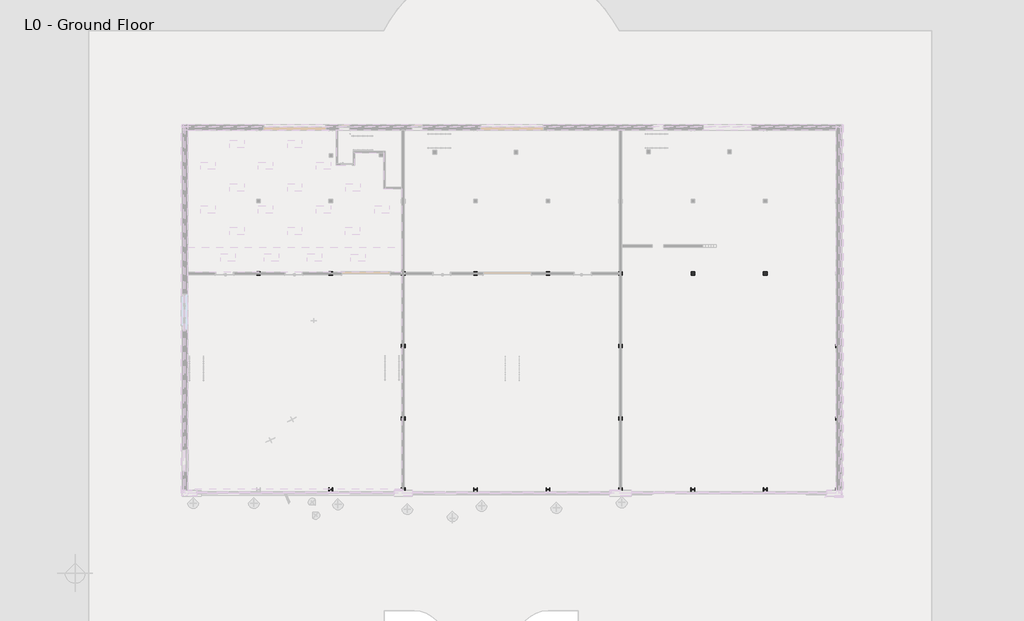
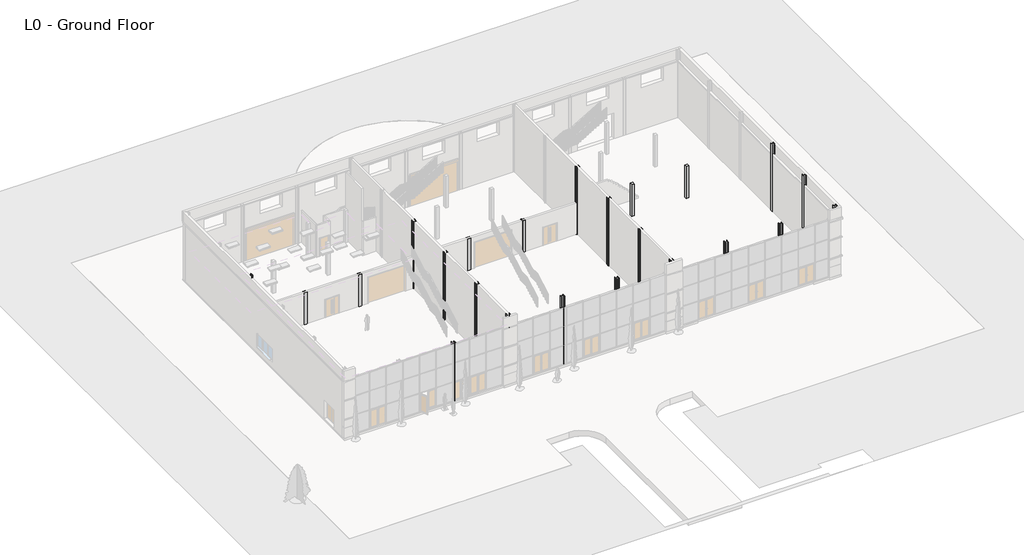
# One storey, part 6 of 14: 23 columns, 22 slabs, 8 footings.
"""IFC4 building model written with IfcOpenShell, lengths in millimetres."""

import ifcopenshell
import ifcopenshell.guid

model = None  # the IFC model being written
_history = None  # IfcOwnerHistory: only IFC2X3 demands one
_inside = {}  # id of a spatial element -> (the spatial element, [elements in it])
_under = {}  # id of a project, library or spatial element -> (it, [spatial elements below it])
_declared = {}  # id of a project -> (the project, [libraries it declares])
_typed = {}  # id of a type object -> (the type object, [elements of that type])
_made_of = {}  # id of a material, layer set ... -> (it, [elements and type objects made of it])


def new_model(schema):
    """Start an empty IFC model of exactly this schema.

    Asked for "IFC4X3", IfcOpenShell would pick the latest addendum, in which some entities
    have other attributes; the version numbers below select the first issue.
    IFC2X3 requires an IfcOwnerHistory on every rooted entity: one is made here for all.
    """
    global model, _history
    if schema == "IFC4X3":
        model = ifcopenshell.file(schema_version=(4, 3, 0, 0))
    else:
        model = ifcopenshell.file(schema=schema)
    _inside.clear()
    _under.clear()
    _declared.clear()
    _typed.clear()
    _made_of.clear()
    _history = None
    if model.schema == "IFC2X3":
        org = make("IfcOrganization", Name="unknown")
        user = make(
            "IfcPersonAndOrganization",
            ThePerson=make("IfcPerson", FamilyName="unknown"),
            TheOrganization=org,
        )
        app = make(
            "IfcApplication",
            ApplicationDeveloper=org,
            Version="unknown",
            ApplicationFullName="unknown",
            ApplicationIdentifier="unknown",
        )
        _history = make(
            "IfcOwnerHistory",
            OwningUser=user,
            OwningApplication=app,
            ChangeAction="ADDED",
            CreationDate=0,
        )
    return model


def make(cls, **values):
    """One entity of the class cls with the attributes given. An attribute that is None is left unset."""
    return model.create_entity(
        cls, **{name: value for name, value in values.items() if value is not None}
    )


def rooted(cls, **values):
    """An entity with a GlobalId (a new one), such as an element, a storey or a relation."""
    return make(cls, GlobalId=ifcopenshell.guid.new(), OwnerHistory=_history, **values)


def si_unit(unit_type, name, prefix=None):
    """IfcSIUnit, for example si_unit("LENGTHUNIT", "METRE", prefix="MILLI")."""
    return make("IfcSIUnit", UnitType=unit_type, Prefix=prefix, Name=name)


def assignment(units):
    """IfcUnitAssignment: the units of a project."""
    return None if units is None else make("IfcUnitAssignment", Units=units)


def point(xyz):
    """IfcCartesianPoint."""
    return None if xyz is None else make("IfcCartesianPoint", Coordinates=xyz)


def direction(xyz):
    """IfcDirection."""
    return None if xyz is None else make("IfcDirection", DirectionRatios=xyz)


def frame(location, z_axis=None, x_axis=None):
    """IfcAxis2Placement3D, a coordinate frame: its origin and axes. An axis left out is left unset."""
    return make(
        "IfcAxis2Placement3D",
        Location=point(location),
        Axis=direction(z_axis),
        RefDirection=direction(x_axis),
    )


def frame_2d(location, x_axis=None):
    """IfcAxis2Placement2D, a coordinate frame in the plane: its origin and x axis."""
    return make(
        "IfcAxis2Placement2D", Location=point(location), RefDirection=direction(x_axis)
    )


def origin():
    """The frame at (0, 0, 0) with its axes left unset."""
    return frame((0.0, 0.0, 0.0))


def place(relative_to, where):
    """IfcLocalPlacement: puts the frame where relative to a parent placement (None: the world)."""
    return make(
        "IfcLocalPlacement", PlacementRelTo=relative_to, RelativePlacement=where
    )


def context(
    kind, dimensions, precision=None, world=None, true_north=None, identifier=None
):
    """IfcGeometricRepresentationContext, for example the 3D "Model" context."""
    return make(
        "IfcGeometricRepresentationContext",
        ContextIdentifier=identifier,
        ContextType=kind,
        CoordinateSpaceDimension=dimensions,
        Precision=precision,
        WorldCoordinateSystem=world,
        TrueNorth=true_north,
    )


def project(units=None, contexts=None):
    """IfcProject with its units and contexts."""
    return rooted(
        "IfcProject",
        Name="project",
        RepresentationContexts=contexts,
        UnitsInContext=assignment(units),
    )


def spatial(cls, under=None, at=None, **own):
    """A site, building, storey or space (cls), placed at a placement, below another one or the project."""
    s = rooted(cls, ObjectPlacement=at, **own)
    if under is not None:
        _under.setdefault(under.id(), (under, []))[1].append(s)
    return s


def polyline(points):
    """IfcPolyline through the points."""
    return make("IfcPolyline", Points=[point(p) for p in points])


def circle_curve(where, radius):
    """IfcCircle in the frame where."""
    return make("IfcCircle", Position=where, Radius=radius)


def trimmed(basis, trim1, trim2, sense, master):
    """IfcTrimmedCurve: the piece of a basis curve between two trims."""
    return make(
        "IfcTrimmedCurve",
        BasisCurve=basis,
        Trim1=trim1,
        Trim2=trim2,
        SenseAgreement=sense,
        MasterRepresentation=master,
    )


def segment(curve, same_sense, transition):
    """IfcCompositeCurveSegment."""
    return make(
        "IfcCompositeCurveSegment",
        Transition=transition,
        SameSense=same_sense,
        ParentCurve=curve,
    )


def composite_curve(segments, self_intersect=None):
    """IfcCompositeCurve: segments joined end to end."""
    return make("IfcCompositeCurve", Segments=segments, SelfIntersect=self_intersect)


def outline(outer, holes=None, kind="AREA"):
    """IfcArbitraryClosedProfileDef: a profile drawn as a closed curve; with holes, ...WithVoids."""
    if holes is None:
        return make("IfcArbitraryClosedProfileDef", ProfileType=kind, OuterCurve=outer)
    return make(
        "IfcArbitraryProfileDefWithVoids",
        ProfileType=kind,
        OuterCurve=outer,
        InnerCurves=holes,
    )


def extrude(swept, where, along, depth):
    """IfcExtrudedAreaSolid: the profile swept, set in the frame where, extruded along a direction by depth."""
    return make(
        "IfcExtrudedAreaSolid",
        SweptArea=swept,
        Position=where,
        ExtrudedDirection=direction(along),
        Depth=depth,
    )


def faces_of(points, faces, orient=None, outer=None):
    """IfcFace entities. A face is a list of loops; a loop is a list of indices into points, from 0.

    orient and outer hold one flag for each loop. By default every Orientation is true, the
    first loop of a face is its IfcFaceOuterBound and the others are IfcFaceBound.
    """
    made = []
    for i, loops in enumerate(faces):
        bounds = []
        for j, loop in enumerate(loops):
            is_outer = j == 0 if outer is None else outer[i][j]
            bounds.append(
                make(
                    "IfcFaceOuterBound" if is_outer else "IfcFaceBound",
                    Bound=make("IfcPolyLoop", Polygon=[points[k] for k in loop]),
                    Orientation=True if orient is None else orient[i][j],
                )
            )
        made.append(make("IfcFace", Bounds=bounds))
    return made


def faceted_brep(points, faces, orient=None, outer=None, voids=None):
    """IfcFacetedBrep: a solid bounded by flat faces; with voids (closed shells), ...WithVoids."""
    shared = [point(p) for p in points]
    hull = make("IfcClosedShell", CfsFaces=faces_of(shared, faces, orient, outer))
    if voids is None:
        return make("IfcFacetedBrep", Outer=hull)
    return make(
        "IfcFacetedBrepWithVoids",
        Outer=hull,
        Voids=[
            make(cls, CfsFaces=faces_of(shared, fs, o, b)) for cls, fs, o, b in voids
        ],
    )


def shape(context_of_items, identifier, shape_type, items):
    """IfcShapeRepresentation: the items that make up one representation, for example the "Body"."""
    return make(
        "IfcShapeRepresentation",
        ContextOfItems=context_of_items,
        RepresentationIdentifier=identifier,
        RepresentationType=shape_type,
        Items=items,
    )


def source(mapping_origin, context_of_items, identifier, shape_type, items):
    """IfcRepresentationMap: a shape defined once, which mapped items show again and again."""
    return make(
        "IfcRepresentationMap",
        MappingOrigin=mapping_origin,
        MappedRepresentation=shape(context_of_items, identifier, shape_type, items),
    )


def transform(
    local_origin,
    x_axis=None,
    y_axis=None,
    z_axis=None,
    scale=None,
    scale2=None,
    scale3=None,
    uniform=True,
):
    """IfcCartesianTransformationOperator3D, or its non-uniform kind. x_axis, y_axis, z_axis: its Axis1, 2, 3."""
    if uniform:
        return make(
            "IfcCartesianTransformationOperator3D",
            Axis1=direction(x_axis),
            Axis2=direction(y_axis),
            LocalOrigin=point(local_origin),
            Scale=scale,
            Axis3=direction(z_axis),
        )
    return make(
        "IfcCartesianTransformationOperator3DnonUniform",
        Axis1=direction(x_axis),
        Axis2=direction(y_axis),
        LocalOrigin=point(local_origin),
        Scale=scale,
        Axis3=direction(z_axis),
        Scale2=scale2,
        Scale3=scale3,
    )


def mapped(mapping_source, mapping_target):
    """IfcMappedItem: shows the shape of a source again, moved by a transform."""
    return make(
        "IfcMappedItem", MappingSource=mapping_source, MappingTarget=mapping_target
    )


def made_of(thing, what):
    """Note that an element or type object is made of a material, layer set ...; save() writes the relation."""
    if what is not None:
        _made_of.setdefault(what.id(), (what, []))[1].append(thing)
    return thing


def element(
    cls,
    number,
    at=None,
    inside=None,
    cuts=None,
    type_object=None,
    material=None,
    context=None,
    identifier="Body",
    shape_type=None,
    held_by="IfcProductDefinitionShape",
    body=None,
    shapes=None,
    **own,
):
    """One element of the class cls, such as IfcWall. Its Tag is "e" and its number.

    at: its placement. inside: the storey or other place that contains it. cuts: it is an
    opening in that element (IfcRelVoidsElement). A single representation is given by context,
    identifier, shape_type and body (its items); several are given by shapes. held_by: the class
    of the entity that holds the representations. save() writes the other relations.
    """
    e = rooted(cls, Tag="e%d" % number, ObjectPlacement=at, **own)
    if body is not None:
        shapes = [shape(context, identifier, shape_type, body)]
    if shapes is not None:
        e.Representation = make(held_by, Representations=shapes)
    if inside is not None:
        _inside.setdefault(inside.id(), (inside, []))[1].append(e)
    if cuts is not None:
        rooted(
            "IfcRelVoidsElement", RelatingBuildingElement=cuts, RelatedOpeningElement=e
        )
    if type_object is not None:
        _typed.setdefault(type_object.id(), (type_object, []))[1].append(e)
    return made_of(e, material)


def aggregate(whole, parts):
    """IfcRelAggregates: a whole, such as a stair, and the parts it consists of."""
    return rooted("IfcRelAggregates", RelatingObject=whole, RelatedObjects=parts)


def save(model, path):
    """Write the relations noted so far, then the file.

    IfcRelAggregates (storeys below a building ...), IfcRelContainedInSpatialStructure (elements
    in a storey), IfcRelDefinesByType, IfcRelAssociatesMaterial and IfcRelDeclares: one each for
    every whole, place, type object, material and project.
    """
    for whole, parts in _under.values():
        aggregate(whole, parts)
    for where, things in _inside.values():
        rooted(
            "IfcRelContainedInSpatialStructure",
            RelatedElements=things,
            RelatingStructure=where,
        )
    for kind, things in _typed.values():
        rooted("IfcRelDefinesByType", RelatedObjects=things, RelatingType=kind)
    for what, things in _made_of.values():
        rooted("IfcRelAssociatesMaterial", RelatedObjects=things, RelatingMaterial=what)
    for by, libraries in _declared.values():
        rooted("IfcRelDeclares", RelatingContext=by, RelatedDefinitions=libraries)
    model.write(path)


def uc_universal_column_column_305x305x97uc_f4bfb62a(model_context):
    return source(origin(), model_context, "Body", "SweptSolid", [
        extrude(outline(composite_curve([segment(polyline([(152.65, 153.95), (152.65, 138.55), (20.15, 138.55)]), True, "CONTINUOUS"), segment(trimmed(circle_curve(frame_2d((20.15, 123.35)), 15.2), [point((20.15, 138.55))], [point((4.95, 123.35))], True, "CARTESIAN"), True, "CONTINUOUS"), segment(polyline([(4.95, 123.35), (4.95, -123.35)]), True, "CONTINUOUS"), segment(trimmed(circle_curve(frame_2d((20.15, -123.35)), 15.2), [point((4.95, -123.35))], [point((20.15, -138.55))], True, "CARTESIAN"), True, "CONTINUOUS"), segment(polyline([(20.15, -138.55), (152.65, -138.55), (152.65, -153.95), (-152.65, -153.95), (-152.65, -138.55), (-20.15, -138.55)]), True, "CONTINUOUS"), segment(trimmed(circle_curve(frame_2d((-20.15, -123.35)), 15.2), [point((-20.15, -138.55))], [point((-4.95, -123.35))], True, "CARTESIAN"), True, "CONTINUOUS"), segment(polyline([(-4.95, -123.35), (-4.95, 123.35)]), True, "CONTINUOUS"), segment(trimmed(circle_curve(frame_2d((-20.15, 123.35)), 15.2), [point((-4.95, 123.35))], [point((-20.15, 138.55))], True, "CARTESIAN"), True, "CONTINUOUS"), segment(polyline([(-20.15, 138.55), (-152.65, 138.55), (-152.65, 153.95), (152.65, 153.95)]), True, "CONTINUOUS")], self_intersect=False)), frame((0.0, 0.0, -1500.0), z_axis=(0.0, 0.0, 1.0), x_axis=(1.0, 0.0, 0.0)), (0.0, 0.0, 1.0), 9300.0),
    ])


def uc_universal_column_column_305x305x97uc_8da79b43(model_context):
    return source(origin(), model_context, "Body", "SweptSolid", [
        extrude(outline(composite_curve([segment(polyline([(152.65, -153.95), (-152.65, -153.95), (-152.65, -138.55), (-20.15, -138.55)]), True, "CONTINUOUS"), segment(trimmed(circle_curve(frame_2d((-20.15, -123.35)), 15.2), [point((-20.15, -138.55))], [point((-4.95, -123.35))], True, "CARTESIAN"), True, "CONTINUOUS"), segment(polyline([(-4.95, -123.35), (-4.95, 123.35)]), True, "CONTINUOUS"), segment(trimmed(circle_curve(frame_2d((-20.15, 123.35)), 15.2), [point((-4.95, 123.35))], [point((-20.15, 138.55))], True, "CARTESIAN"), True, "CONTINUOUS"), segment(polyline([(-20.15, 138.55), (-152.65, 138.55), (-152.65, 153.95), (152.65, 153.95), (152.65, 138.55), (20.15, 138.55)]), True, "CONTINUOUS"), segment(trimmed(circle_curve(frame_2d((20.15, 123.35)), 15.2), [point((20.15, 138.55))], [point((4.95, 123.35))], True, "CARTESIAN"), True, "CONTINUOUS"), segment(polyline([(4.95, 123.35), (4.95, -123.35)]), True, "CONTINUOUS"), segment(trimmed(circle_curve(frame_2d((20.15, -123.35)), 15.2), [point((4.95, -123.35))], [point((20.15, -138.55))], True, "CARTESIAN"), True, "CONTINUOUS"), segment(polyline([(20.15, -138.55), (152.65, -138.55), (152.65, -153.95)]), True, "CONTINUOUS")], self_intersect=False)), frame((0.0, 0.0, -1500.0), z_axis=(0.0, 0.0, 1.0), x_axis=(1.0, 0.0, 0.0)), (0.0, 0.0, 1.0), 9300.0),
    ])


def uc_universal_column_column_305x305x97uc_43a052ce(model_context):
    return source(origin(), model_context, "Body", "SweptSolid", [
        extrude(outline(composite_curve([segment(polyline([(152.65, 153.95), (152.65, 138.55), (20.15, 138.55)]), True, "CONTINUOUS"), segment(trimmed(circle_curve(frame_2d((20.15, 123.35)), 15.2), [point((20.15, 138.55))], [point((4.95, 123.35))], True, "CARTESIAN"), True, "CONTINUOUS"), segment(polyline([(4.95, 123.35), (4.95, -123.35)]), True, "CONTINUOUS"), segment(trimmed(circle_curve(frame_2d((20.15, -123.35)), 15.2), [point((4.95, -123.35))], [point((20.15, -138.55))], True, "CARTESIAN"), True, "CONTINUOUS"), segment(polyline([(20.15, -138.55), (152.65, -138.55), (152.65, -153.95), (-152.65, -153.95), (-152.65, -138.55), (-20.15, -138.55)]), True, "CONTINUOUS"), segment(trimmed(circle_curve(frame_2d((-20.15, -123.35)), 15.2), [point((-20.15, -138.55))], [point((-4.95, -123.35))], True, "CARTESIAN"), True, "CONTINUOUS"), segment(polyline([(-4.95, -123.35), (-4.95, 123.35)]), True, "CONTINUOUS"), segment(trimmed(circle_curve(frame_2d((-20.15, 123.35)), 15.2), [point((-4.95, 123.35))], [point((-20.15, 138.55))], True, "CARTESIAN"), True, "CONTINUOUS"), segment(polyline([(-20.15, 138.55), (-152.65, 138.55), (-152.65, 153.95), (152.65, 153.95)]), True, "CONTINUOUS")], self_intersect=False)), frame((0.0, 0.0, -1500.0), z_axis=(0.0, 0.0, 1.0), x_axis=(1.0, 0.0, 0.0)), (0.0, 0.0, 1.0), 8100.0),
    ])


def pad_foundation_rectangular_1000x1000x500_ed6229e9(model_context):
    return source(origin(), model_context, "Body", "SweptSolid", [
        extrude(outline(polyline([(500.0, 500.0), (500.0, -500.0), (-500.0, -500.0), (-500.0, 500.0), (500.0, 500.0)])), frame((0.0, 0.0, -500.0), z_axis=(0.0, 0.0, 1.0), x_axis=(1.0, 0.0, 0.0)), (0.0, 0.0, 1.0), 500.0),
    ])


model = new_model("IFC4")

# Units and contexts
model_context = context("Model", 3, world=origin())
ifc_project = project(units=[si_unit("LENGTHUNIT", "METRE", prefix="MILLI")], contexts=[model_context])

# Site, building, storey
site = spatial("IfcSite", under=ifc_project)
building = spatial("IfcBuilding", under=site)
storey = spatial("IfcBuildingStorey", under=building, Name="L0 - Ground Floor", Elevation=0.0)

# Columns
placement = place(None, origin())
element("IfcColumn", 1, ObjectType="Concrete Square : 300 x 300mm", at=placement, inside=storey, context=model_context, shape_type="SweptSolid", body=[
    extrude(outline(polyline([(-989.5553457, -5208.7619082), (-1289.5553457, -5208.7619082), (-1289.5553457, -4908.7619082), (-989.5553457, -4908.7619082), (-989.5553457, -5208.7619082)])), frame((0.0, 0.0, -1500.0), z_axis=(0.0, 0.0, 1.0), x_axis=(1.0, 0.0, 0.0)), (0.0, 0.0, 1.0), 5200.0),
])
element("IfcColumn", 2, ObjectType="Concrete Square : 300 x 300mm", at=placement, inside=storey, context=model_context, shape_type="SweptSolid", body=[
    extrude(outline(polyline([(5010.4446543, -5208.7619082), (4710.4446543, -5208.7619082), (4710.4446543, -4908.7619082), (5010.4446543, -4908.7619082), (5010.4446543, -5208.7619082)])), frame((0.0, 0.0, -1500.0), z_axis=(0.0, 0.0, 1.0), x_axis=(1.0, 0.0, 0.0)), (0.0, 0.0, 1.0), 5200.0),
])
element("IfcColumn", 3, ObjectType="Concrete Square : 300 x 300mm", at=placement, inside=storey, context=model_context, shape_type="SweptSolid", body=[
    extrude(outline(polyline([(17010.4446543, -5208.7619082), (16710.4446543, -5208.7619082), (16710.4446543, -4908.7619082), (17010.4446543, -4908.7619082), (17010.4446543, -5208.7619082)])), frame((0.0, 0.0, -1500.0), z_axis=(0.0, 0.0, 1.0), x_axis=(1.0, 0.0, 0.0)), (0.0, 0.0, 1.0), 5200.0),
])
element("IfcColumn", 4, ObjectType="Concrete Square : 300 x 300mm", at=placement, inside=storey, context=model_context, shape_type="SweptSolid", body=[
    extrude(outline(polyline([(23010.4446543, -5208.7619082), (22710.4446543, -5208.7619082), (22710.4446543, -4908.7619082), (23010.4446543, -4908.7619082), (23010.4446543, -5208.7619082)])), frame((0.0, 0.0, -1500.0), z_axis=(0.0, 0.0, 1.0), x_axis=(1.0, 0.0, 0.0)), (0.0, 0.0, 1.0), 5200.0),
])
element("IfcColumn", 5, ObjectType="Concrete Square : 300 x 300mm", at=placement, inside=storey, context=model_context, shape_type="SweptSolid", body=[
    extrude(outline(polyline([(35010.4446543, -5208.7619082), (34710.4446543, -5208.7619082), (34710.4446543, -4908.7619082), (35010.4446543, -4908.7619082), (35010.4446543, -5208.7619082)])), frame((0.0, 0.0, -1500.0), z_axis=(0.0, 0.0, 1.0), x_axis=(1.0, 0.0, 0.0)), (0.0, 0.0, 1.0), 5200.0),
])
element("IfcColumn", 6, ObjectType="Concrete Square : 300 x 300mm", at=placement, inside=storey, context=model_context, shape_type="SweptSolid", body=[
    extrude(outline(polyline([(41010.4446543, -5208.7619082), (40710.4446543, -5208.7619082), (40710.4446543, -4908.7619082), (41010.4446543, -4908.7619082), (41010.4446543, -5208.7619082)])), frame((0.0, 0.0, -1500.0), z_axis=(0.0, 0.0, 1.0), x_axis=(1.0, 0.0, 0.0)), (0.0, 0.0, 1.0), 5200.0),
])
element("IfcColumn", 7, ObjectType="UC-Universal Column-Column : 305x305x97UC", at=placement, inside=storey, context=model_context, shape_type="SweptSolid", body=[
    extrude(outline(composite_curve([segment(polyline([(-7293.5053457, -4906.1119082), (-7278.1053457, -4906.1119082), (-7278.1053457, -5038.6119082)]), True, "CONTINUOUS"), segment(trimmed(circle_curve(frame_2d((-7262.9053457, -5038.6119082)), 15.2), [point((-7278.1053457, -5038.6119082))], [point((-7262.9053457, -5053.8119082))], True, "CARTESIAN"), True, "CONTINUOUS"), segment(polyline([(-7262.9053457, -5053.8119082), (-7016.2053457, -5053.8119082)]), True, "CONTINUOUS"), segment(trimmed(circle_curve(frame_2d((-7016.2053457, -5038.6119082)), 15.2), [point((-7016.2053457, -5053.8119082))], [point((-7001.0053457, -5038.6119082))], True, "CARTESIAN"), True, "CONTINUOUS"), segment(polyline([(-7001.0053457, -5038.6119082), (-7001.0053457, -4906.1119082), (-6985.6053457, -4906.1119082), (-6985.6053457, -5211.4119082), (-7001.0053457, -5211.4119082), (-7001.0053457, -5078.9119082)]), True, "CONTINUOUS"), segment(trimmed(circle_curve(frame_2d((-7016.2053457, -5078.9119082)), 15.2), [point((-7001.0053457, -5078.9119082))], [point((-7016.2053457, -5063.7119082))], True, "CARTESIAN"), True, "CONTINUOUS"), segment(polyline([(-7016.2053457, -5063.7119082), (-7262.9053457, -5063.7119082)]), True, "CONTINUOUS"), segment(trimmed(circle_curve(frame_2d((-7262.9053457, -5078.9119082)), 15.2), [point((-7262.9053457, -5063.7119082))], [point((-7278.1053457, -5078.9119082))], True, "CARTESIAN"), True, "CONTINUOUS"), segment(polyline([(-7278.1053457, -5078.9119082), (-7278.1053457, -5211.4119082), (-7293.5053457, -5211.4119082), (-7293.5053457, -4906.1119082)]), True, "CONTINUOUS")], self_intersect=False)), frame((0.0, 0.0, -1500.0), z_axis=(0.0, 0.0, 1.0), x_axis=(1.0, 0.0, 0.0)), (0.0, 0.0, 1.0), 9300.0),
])
uc_universal_column_column_305x305x97uc_shape = uc_universal_column_column_305x305x97uc_f4bfb62a(model_context)
element("IfcColumn", 8, ObjectType="UC-Universal Column-Column : 305x305x97UC", at=placement, inside=storey, context=model_context, shape_type="MappedRepresentation", body=[
    mapped(uc_universal_column_column_305x305x97uc_shape, transform((10860.4446543, -17058.7619082, 0.0), x_axis=(0.0, 1.0, 0.0), y_axis=(-1.0, 0.0, 0.0), z_axis=(0.0, 0.0, 1.0))),
])
element("IfcColumn", 9, ObjectType="UC-Universal Column-Column : 305x305x97UC", at=placement, inside=storey, context=model_context, shape_type="MappedRepresentation", body=[
    mapped(uc_universal_column_column_305x305x97uc_shape, transform((28860.4446543, -17058.7619082, 0.0), x_axis=(0.0, 1.0, 0.0), y_axis=(-1.0, 0.0, 0.0), z_axis=(0.0, 0.0, 1.0))),
])
element("IfcColumn", 10, ObjectType="UC-Universal Column-Column : 305x305x97UC", at=placement, inside=storey, context=model_context, shape_type="MappedRepresentation", body=[
    mapped(uc_universal_column_column_305x305x97uc_shape, transform((10860.4446543, -11058.7619082, 0.0), x_axis=(0.0, 1.0, 0.0), y_axis=(-1.0, 0.0, 0.0), z_axis=(0.0, 0.0, 1.0))),
])
element("IfcColumn", 11, ObjectType="UC-Universal Column-Column : 305x305x97UC", at=placement, inside=storey, context=model_context, shape_type="MappedRepresentation", body=[
    mapped(uc_universal_column_column_305x305x97uc_shape, transform((28860.4446543, -11058.7619082, 0.0), x_axis=(0.0, 1.0, 0.0), y_axis=(-1.0, 0.0, 0.0), z_axis=(0.0, 0.0, 1.0))),
])
element("IfcColumn", 12, ObjectType="UC-Universal Column-Column : 305x305x97UC", at=placement, inside=storey, context=model_context, shape_type="MappedRepresentation", body=[
    mapped(uc_universal_column_column_305x305x97uc_shape, transform((10860.4446543, -5058.7619082, 0.0), x_axis=(0.0, 1.0, 0.0), y_axis=(-1.0, 0.0, 0.0), z_axis=(0.0, 0.0, 1.0))),
])
element("IfcColumn", 13, ObjectType="UC-Universal Column-Column : 305x305x97UC", at=placement, inside=storey, context=model_context, shape_type="MappedRepresentation", body=[
    mapped(uc_universal_column_column_305x305x97uc_shape, transform((28860.4446543, -5058.7619082, 0.0), x_axis=(0.0, 1.0, 0.0), y_axis=(-1.0, 0.0, 0.0), z_axis=(0.0, 0.0, 1.0))),
])
element("IfcColumn", 14, ObjectType="UC-Universal Column-Column : 305x305x97UC", at=placement, inside=storey, context=model_context, shape_type="MappedRepresentation", body=[
    mapped(uc_universal_column_column_305x305x97uc_shape, transform((10860.4446543, -22948.7619082, 0.0), x_axis=(0.0, 1.0, 0.0), y_axis=(-1.0, 0.0, 0.0), z_axis=(0.0, 0.0, 1.0))),
])
element("IfcColumn", 15, ObjectType="UC-Universal Column-Column : 305x305x97UC", at=placement, inside=storey, context=model_context, shape_type="MappedRepresentation", body=[
    mapped(uc_universal_column_column_305x305x97uc_shape, transform((16860.4446543, -22948.7619082, 0.0), x_axis=(0.0, 1.0, 0.0), y_axis=(-1.0, 0.0, 0.0), z_axis=(0.0, 0.0, 1.0))),
])
element("IfcColumn", 16, ObjectType="UC-Universal Column-Column : 305x305x97UC", at=placement, inside=storey, context=model_context, shape_type="MappedRepresentation", body=[
    mapped(uc_universal_column_column_305x305x97uc_shape, transform((22860.4446543, -22948.7619082, 0.0), x_axis=(0.0, 1.0, 0.0), y_axis=(-1.0, 0.0, 0.0), z_axis=(0.0, 0.0, 1.0))),
])
element("IfcColumn", 17, ObjectType="UC-Universal Column-Column : 305x305x97UC", at=placement, inside=storey, context=model_context, shape_type="MappedRepresentation", body=[
    mapped(uc_universal_column_column_305x305x97uc_shape, transform((34860.4446543, -22948.7619082, 0.0), x_axis=(0.0, 1.0, 0.0), y_axis=(-1.0, 0.0, 0.0), z_axis=(0.0, 0.0, 1.0))),
])
element("IfcColumn", 18, ObjectType="UC-Universal Column-Column : 305x305x97UC", at=placement, inside=storey, context=model_context, shape_type="MappedRepresentation", body=[
    mapped(uc_universal_column_column_305x305x97uc_shape, transform((28860.4446543, -22948.7619082, 0.0), x_axis=(0.0, 1.0, 0.0), y_axis=(-1.0, 0.0, 0.0), z_axis=(0.0, 0.0, 1.0))),
])
element("IfcColumn", 19, ObjectType="UC-Universal Column-Column : 305x305x97UC", at=placement, inside=storey, context=model_context, shape_type="MappedRepresentation", body=[
    mapped(uc_universal_column_column_305x305x97uc_shape, transform((40860.4446543, -22948.7619082, 0.0), x_axis=(0.0, 1.0, 0.0), y_axis=(-1.0, 0.0, 0.0), z_axis=(0.0, 0.0, 1.0))),
])
uc_universal_column_column_305x305x97uc_2_shape = uc_universal_column_column_305x305x97uc_8da79b43(model_context)
element("IfcColumn", 20, ObjectType="UC-Universal Column-Column : 305x305x97UC", at=placement, inside=storey, context=model_context, shape_type="MappedRepresentation", body=[
    mapped(uc_universal_column_column_305x305x97uc_2_shape, transform((46860.4446543, -22948.7619082, 0.0), x_axis=(0.0, 1.0, 0.0), y_axis=(-1.0, 0.0, 0.0), z_axis=(0.0, 0.0, 1.0))),
])
element("IfcColumn", 21, ObjectType="UC-Universal Column-Column : 305x305x97UC", at=placement, inside=storey, context=model_context, shape_type="MappedRepresentation", body=[
    mapped(uc_universal_column_column_305x305x97uc_2_shape, transform((46860.4446543, -17058.7619082, 0.0), x_axis=(0.0, 1.0, 0.0), y_axis=(-1.0, 0.0, 0.0), z_axis=(0.0, 0.0, 1.0))),
])
element("IfcColumn", 22, ObjectType="UC-Universal Column-Column : 305x305x97UC", at=placement, inside=storey, context=model_context, shape_type="MappedRepresentation", body=[
    mapped(uc_universal_column_column_305x305x97uc_2_shape, transform((46860.4446543, -11058.7619082, 0.0), x_axis=(0.0, 1.0, 0.0), y_axis=(-1.0, 0.0, 0.0), z_axis=(0.0, 0.0, 1.0))),
])
uc_universal_column_column_305x305x97uc_3_shape = uc_universal_column_column_305x305x97uc_43a052ce(model_context)
element("IfcColumn", 23, ObjectType="UC-Universal Column-Column : 305x305x97UC", at=placement, inside=storey, context=model_context, shape_type="MappedRepresentation", body=[
    mapped(uc_universal_column_column_305x305x97uc_3_shape, transform((4860.4446543, -22948.7619082, 0.0), x_axis=(0.0, 1.0, 0.0), y_axis=(-1.0, 0.0, 0.0), z_axis=(0.0, 0.0, 1.0))),
])

# Footings
element("IfcFooting", 24, ObjectType="Wall Foundation - Commercial 1300 x 450", at=placement, inside=storey, context=model_context, shape_type="Brep", body=[
    faceted_brep([(-7673.2053457, 7505.9380918, -1200.0), (-7673.2053457, -23738.4619082, -1200.0), (-6758.8053457, -23738.4619082, -1200.0), (-6758.8053457, -22824.0619082, -1200.0), (-6758.8053457, 6591.5380918, -1200.0), (-6758.8053457, 7505.9380918, -1200.0), (-7673.2053457, 7505.9380918, -1504.8), (-7673.2053457, -23738.4619082, -1504.8), (-6758.8053457, 7505.9380918, -1504.8), (-6758.8053457, 7441.2380918, -1504.8), (-7639.5553457, 7441.2380918, -1504.8), (-7639.5553457, 6441.2380918, -1504.8), (-6758.8053457, 6441.2380918, -1504.8), (-6758.8053457, 1441.2380918, -1504.8), (-7639.5553457, 1441.2380918, -1504.8), (-7639.5553457, 441.2380918, -1504.8), (-6758.8053457, 441.2380918, -1504.8), (-6758.8053457, -4558.7619082, -1504.8), (-7639.5553457, -4558.7619082, -1504.8), (-7639.5553457, -5558.7619082, -1504.8), (-6758.8053457, -5558.7619082, -1504.8), (-6758.8053457, -10558.7619082, -1504.8), (-7639.5553457, -10558.7619082, -1504.8), (-7639.5553457, -11558.7619082, -1504.8), (-6758.8053457, -11558.7619082, -1504.8), (-6758.8053457, -16558.7619082, -1504.8), (-7639.5553457, -16558.7619082, -1504.8), (-7639.5553457, -17558.7619082, -1504.8), (-6758.8053457, -17558.7619082, -1504.8), (-6758.8053457, -22448.7619082, -1504.8), (-7639.5553457, -22448.7619082, -1504.8), (-7639.5553457, -23448.7619082, -1504.8), (-6758.8053457, -23448.7619082, -1504.8), (-6758.8053457, -23738.4619082, -1504.8), (-6758.8053457, -23448.7619082, -1500.0), (-6758.8053457, -22824.0619082, -1500.0), (-6758.8053457, -22448.7619082, -1500.0), (-6758.8053457, -17558.7619082, -1500.0), (-6758.8053457, -16558.7619082, -1500.0), (-6758.8053457, -11558.7619082, -1500.0), (-6758.8053457, -10558.7619082, -1500.0), (-6758.8053457, -5558.7619082, -1500.0), (-6758.8053457, -4558.7619082, -1500.0), (-6758.8053457, 441.2380918, -1500.0), (-6758.8053457, 1441.2380918, -1500.0), (-6758.8053457, 6441.2380918, -1500.0), (-6758.8053457, 6591.5380918, -1500.0), (-6758.8053457, 7441.2380918, -1500.0), (-7639.5553457, 441.2380918, -1500.0), (-7639.5553457, 1441.2380918, -1500.0), (-7639.5553457, 6441.2380918, -1500.0), (-7639.5553457, 7441.2380918, -1500.0), (-7639.5553457, -5558.7619082, -1500.0), (-7639.5553457, -4558.7619082, -1500.0), (-7639.5553457, -11558.7619082, -1500.0), (-7639.5553457, -10558.7619082, -1500.0), (-7639.5553457, -17558.7619082, -1500.0), (-7639.5553457, -16558.7619082, -1500.0), (-7639.5553457, -23448.7619082, -1500.0), (-7639.5553457, -22448.7619082, -1500.0)], [[[0, 1, 2, 3, 4, 5]], [[1, 0, 6, 7]], [[7, 6, 8, 9, 10, 11, 12, 13, 14, 15, 16, 17, 18, 19, 20, 21, 22, 23, 24, 25, 26, 27, 28, 29, 30, 31, 32, 33]], [[5, 4, 3, 2, 33, 32, 34, 35, 36, 29, 28, 37, 38, 25, 24, 39, 40, 21, 20, 41, 42, 17, 16, 43, 44, 13, 12, 45, 46, 47, 9, 8]], [[2, 1, 7, 33]], [[48, 49, 44, 43]], [[44, 49, 14, 13]], [[49, 48, 15, 14]], [[48, 43, 16, 15]], [[50, 51, 47, 46, 45]], [[51, 50, 11, 10]], [[50, 45, 12, 11]], [[52, 53, 42, 41]], [[42, 53, 18, 17]], [[53, 52, 19, 18]], [[52, 41, 20, 19]], [[54, 55, 40, 39]], [[40, 55, 22, 21]], [[55, 54, 23, 22]], [[54, 39, 24, 23]], [[56, 57, 38, 37]], [[38, 57, 26, 25]], [[57, 56, 27, 26]], [[56, 37, 28, 27]], [[58, 59, 36, 35, 34]], [[36, 59, 30, 29]], [[59, 58, 31, 30]], [[0, 5, 8, 6]], [[47, 51, 10, 9]], [[58, 34, 32, 31]]]),
])
element("IfcFooting", 25, ObjectType="Wall Foundation - Commercial 1300 x 450", at=placement, inside=storey, context=model_context, shape_type="Brep", body=[
    faceted_brep([(11600.0976476, -23733.4474846, -1200.0), (11600.0976476, -23733.4474846, -1504.8), (11600.0976476, -23618.4474846, -1504.8), (11600.0976476, -22819.0474846, -1504.8), (11600.0976476, -22819.0474846, -1200.0), (11600.0976476, -23618.4474846, -1200.0), (10120.0976476, -23733.4474846, -1504.8), (10120.0976476, -23733.4474846, -1200.0), (10120.0976476, -23625.2469755, -1200.0), (10120.0976476, -22819.0474846, -1200.0), (10120.0976476, -22819.0474846, -1504.8), (10120.0976476, -23625.2469755, -1504.8), (11317.6446543, -22819.0474846, -1200.0), (10403.2446543, -22819.0474846, -1200.0), (10360.4446543, -22819.0474846, -1504.8), (10360.4446543, -23448.7619082, -1504.8), (11360.4446543, -23448.7619082, -1504.8), (11360.4446543, -22819.0474846, -1504.8), (11360.4446543, -22819.0474846, -1500.0), (11317.6446543, -22819.0474846, -1500.0), (10403.2446543, -22819.0474846, -1500.0), (10360.4446543, -22819.0474846, -1500.0), (11360.4446543, -23448.7619082, -1500.0), (10360.4446543, -23448.7619082, -1500.0)], [[[0, 1, 2, 3, 4, 5]], [[6, 7, 8, 9, 10, 11]], [[7, 0, 5, 4, 12, 13, 9, 8]], [[1, 0, 7, 6]], [[3, 2, 1, 6, 11, 10, 14, 15, 16, 17]], [[4, 3, 17, 18, 19, 20, 21, 14, 10, 9, 13, 12]], [[22, 23, 21, 20, 19, 18]], [[21, 23, 15, 14]], [[23, 22, 16, 15]], [[22, 18, 17, 16]]]),
])
element("IfcFooting", 26, ObjectType="Wall Foundation - Commercial 1300 x 450", at=placement, inside=storey, context=model_context, shape_type="Brep", body=[
    faceted_brep([(31560.0976476, -23733.4474846, -1200.0), (31560.0976476, -23733.4474846, -1504.8), (31560.0976476, -22819.0474846, -1504.8), (31560.0976476, -22819.0474846, -1200.0), (27960.0976476, -23733.4474846, -1504.8), (27960.0976476, -23733.4474846, -1200.0), (27960.0976476, -23618.4474846, -1200.0), (27960.0976476, -22819.0474846, -1200.0), (27960.0976476, -22819.0474846, -1504.8), (27960.0976476, -23618.4474846, -1504.8), (29317.6446543, -22819.0474846, -1200.0), (28403.2446543, -22819.0474846, -1200.0), (28360.4446543, -22819.0474846, -1504.8), (28360.4446543, -23448.7619082, -1504.8), (29360.4446543, -23448.7619082, -1504.8), (29360.4446543, -22819.0474846, -1504.8), (29360.4446543, -22819.0474846, -1500.0), (29317.6446543, -22819.0474846, -1500.0), (28403.2446543, -22819.0474846, -1500.0), (28360.4446543, -22819.0474846, -1500.0), (29360.4446543, -23448.7619082, -1500.0), (28360.4446543, -23448.7619082, -1500.0)], [[[0, 1, 2, 3]], [[4, 5, 6, 7, 8, 9]], [[5, 0, 3, 10, 11, 7, 6]], [[1, 0, 5, 4]], [[2, 1, 4, 9, 8, 12, 13, 14, 15]], [[3, 2, 15, 16, 17, 18, 19, 12, 8, 7, 11, 10]], [[20, 21, 19, 18, 17, 16]], [[19, 21, 13, 12]], [[21, 20, 14, 13]], [[20, 16, 15, 14]]]),
])
element("IfcFooting", 27, ObjectType="Wall Foundation - Commercial 1300 x 450", at=placement, inside=storey, context=model_context, shape_type="Brep", body=[
    faceted_brep([(43960.0976476, -23733.4474846, -1504.8), (43960.0976476, -23733.4474846, -1200.0), (43960.0976476, -22819.0474846, -1200.0), (43960.0976476, -22819.0474846, -1504.8), (47425.1446543, -23733.4474846, -1200.0), (47425.1446543, -22819.0474846, -1200.0), (46510.7446543, -22819.0474846, -1200.0), (47425.1446543, -23733.4474846, -1504.8), (46360.4446543, -22819.0474846, -1504.8), (46360.4446543, -23448.7619082, -1504.8), (47360.4446543, -23448.7619082, -1504.8), (47360.4446543, -22819.0474846, -1504.8), (47425.1446543, -22819.0474846, -1504.8), (47360.4446543, -22819.0474846, -1500.0), (46510.7446543, -22819.0474846, -1500.0), (46360.4446543, -22819.0474846, -1500.0), (47360.4446543, -23448.7619082, -1500.0), (46360.4446543, -23448.7619082, -1500.0)], [[[0, 1, 2, 3]], [[1, 4, 5, 6, 2]], [[1, 0, 7, 4]], [[0, 3, 8, 9, 10, 11, 12, 7]], [[3, 2, 6, 5, 12, 11, 13, 14, 15, 8]], [[16, 17, 15, 14, 13]], [[15, 17, 9, 8]], [[17, 16, 10, 9]], [[5, 4, 7, 12]], [[16, 13, 11, 10]]]),
])
element("IfcFooting", 28, ObjectType="Wall Foundation - Commercial 1300 x 450", at=placement, inside=storey, context=model_context, shape_type="SweptSolid", body=[
    extrude(outline(polyline([(1441.2380918, -1500.0), (441.2380918, -1500.0), (441.2380918, -1504.8), (-4558.7619082, -1504.8), (-4558.7619082, -1500.0), (-5558.7619082, -1500.0), (-5558.7619082, -1504.8), (-10558.7619082, -1504.8), (-10558.7619082, -1500.0), (-11558.7619082, -1500.0), (-11558.7619082, -1504.8), (-16558.7619082, -1504.8), (-16558.7619082, -1500.0), (-17558.7619082, -1500.0), (-17558.7619082, -1504.8), (-22448.7619082, -1504.8), (-22448.7619082, -1500.0), (-22819.0474846, -1500.0), (-22819.0474846, -1200.0), (6591.5380918, -1200.0), (6591.5380918, -1500.0), (6441.2380918, -1500.0), (6441.2380918, -1504.8), (1441.2380918, -1504.8), (1441.2380918, -1500.0)])), frame((28403.2446543, 0.0, 0.0), z_axis=(1.0, 0.0, 0.0), x_axis=(0.0, 1.0, 0.0)), (0.0, 0.0, 1.0), 914.4),
])
element("IfcFooting", 29, ObjectType="Wall Foundation - Commercial 1300 x 450", at=placement, inside=storey, context=model_context, shape_type="SweptSolid", body=[
    extrude(outline(polyline([(1441.2380918, -1500.0), (441.2380918, -1500.0), (441.2380918, -1504.8), (-4558.7619082, -1504.8), (-4558.7619082, -1500.0), (-5558.7619082, -1500.0), (-5558.7619082, -1504.8), (-10558.7619082, -1504.8), (-10558.7619082, -1500.0), (-11558.7619082, -1500.0), (-11558.7619082, -1504.8), (-16558.7619082, -1504.8), (-16558.7619082, -1500.0), (-17558.7619082, -1500.0), (-17558.7619082, -1504.8), (-22448.7619082, -1504.8), (-22448.7619082, -1500.0), (-22819.0474846, -1500.0), (-22819.0474846, -1200.0), (6591.5380918, -1200.0), (6591.5380918, -1500.0), (6441.2380918, -1500.0), (6441.2380918, -1504.8), (1441.2380918, -1504.8), (1441.2380918, -1500.0)])), frame((10403.2446543, 0.0, 0.0), z_axis=(1.0, 0.0, 0.0), x_axis=(0.0, 1.0, 0.0)), (0.0, 0.0, 1.0), 914.4),
])
element("IfcFooting", 30, ObjectType="Wall Foundation - Commercial 1300 x 450", at=placement, inside=storey, context=model_context, shape_type="Brep", body=[
    faceted_brep([(-6531.0053457, -22710.8469755, -1200.0), (-6531.0053457, -22710.8469755, -1504.8), (-6531.0053457, -22824.0619082, -1504.8), (-6531.0053457, -23625.2469755, -1504.8), (-6531.0053457, -23625.2469755, -1200.0), (-6531.0053457, -22824.0619082, -1200.0), (10120.0976476, -22710.8469755, -1504.8), (10120.0976476, -22710.8469755, -1200.0), (10120.0976476, -22819.0474846, -1200.0), (10120.0976476, -23625.2469755, -1200.0), (10120.0976476, -23625.2469755, -1504.8), (10120.0976476, -22819.0474846, -1504.8), (-6239.5553457, -23625.2469755, -1200.0), (-6214.1553457, -23625.2469755, -1200.0), (-6214.1553457, -22824.0619082, -1200.0), (-5856.0053457, -22824.0619082, -1200.0), (-5856.0053457, -23625.2469755, -1200.0), (5360.4446543, -22710.8469755, -1504.8), (5360.4446543, -22710.8469755, -1500.0), (4360.4446543, -22710.8469755, -1500.0), (4360.4446543, -22710.8469755, -1504.8), (-639.5553457, -22710.8469755, -1504.8), (-639.5553457, -22710.8469755, -1500.0), (-1639.5553457, -22710.8469755, -1500.0), (-1639.5553457, -22710.8469755, -1504.8), (-1639.5553457, -23448.7619082, -1504.8), (-639.5553457, -23448.7619082, -1504.8), (4360.4446543, -23448.7619082, -1504.8), (5360.4446543, -23448.7619082, -1504.8), (-5856.0053457, -23625.2469755, -1504.8), (-5856.0053457, -22824.0619082, -1504.8), (-6214.1553457, -22824.0619082, -1504.8), (-6214.1553457, -23625.2469755, -1504.8), (-6239.5553457, -23625.2469755, -1504.8), (5360.4446543, -23448.7619082, -1500.0), (4360.4446543, -23448.7619082, -1500.0), (-639.5553457, -23448.7619082, -1500.0), (-1639.5553457, -23448.7619082, -1500.0)], [[[0, 1, 2, 3, 4, 5]], [[6, 7, 8, 9, 10, 11]], [[7, 0, 5, 4, 12, 13, 14, 15, 16, 9, 8]], [[1, 0, 7, 6, 17, 18, 19, 20, 21, 22, 23, 24]], [[3, 2, 1, 24, 25, 26, 21, 20, 27, 28, 17, 6, 11, 10, 29, 30, 31, 32, 33]], [[10, 9, 16, 29]], [[4, 3, 33, 32, 13, 12]], [[34, 35, 19, 18]], [[19, 35, 27, 20]], [[35, 34, 28, 27]], [[34, 18, 17, 28]], [[36, 37, 23, 22]], [[23, 37, 25, 24]], [[37, 36, 26, 25]], [[36, 22, 21, 26]], [[15, 30, 29, 16]], [[30, 15, 14, 31]], [[31, 14, 13, 32]]]),
])
element("IfcFooting", 31, ObjectType="Wall Foundation - Commercial 1300 x 450", at=placement, inside=storey, context=model_context, shape_type="Brep", body=[
    faceted_brep([(27960.0976476, -23618.4474846, -1200.0), (27960.0976476, -23618.4474846, -1504.8), (27960.0976476, -22819.0474846, -1504.8), (27960.0976476, -22704.0474846, -1504.8), (27960.0976476, -22704.0474846, -1200.0), (27960.0976476, -22819.0474846, -1200.0), (11600.0976476, -23618.4474846, -1504.8), (11600.0976476, -23618.4474846, -1200.0), (11600.0976476, -22819.0474846, -1200.0), (11600.0976476, -22704.0474846, -1200.0), (11600.0976476, -22704.0474846, -1504.8), (11600.0976476, -22819.0474846, -1504.8), (16360.4446543, -22704.0474846, -1504.8), (16360.4446543, -23448.7619082, -1504.8), (17360.4446543, -23448.7619082, -1504.8), (17360.4446543, -22704.0474846, -1504.8), (22360.4446543, -22704.0474846, -1504.8), (22360.4446543, -23448.7619082, -1504.8), (23360.4446543, -23448.7619082, -1504.8), (23360.4446543, -22704.0474846, -1504.8), (23360.4446543, -22704.0474846, -1500.0), (22360.4446543, -22704.0474846, -1500.0), (17360.4446543, -22704.0474846, -1500.0), (16360.4446543, -22704.0474846, -1500.0), (23360.4446543, -23448.7619082, -1500.0), (22360.4446543, -23448.7619082, -1500.0), (17360.4446543, -23448.7619082, -1500.0), (16360.4446543, -23448.7619082, -1500.0)], [[[0, 1, 2, 3, 4, 5]], [[6, 7, 8, 9, 10, 11]], [[7, 0, 5, 4, 9, 8]], [[1, 0, 7, 6]], [[3, 2, 1, 6, 11, 10, 12, 13, 14, 15, 16, 17, 18, 19]], [[4, 3, 19, 20, 21, 16, 15, 22, 23, 12, 10, 9]], [[24, 25, 21, 20]], [[21, 25, 17, 16]], [[25, 24, 18, 17]], [[24, 20, 19, 18]], [[26, 27, 23, 22]], [[23, 27, 13, 12]], [[27, 26, 14, 13]], [[26, 22, 15, 14]]]),
])

# Slabs
element("IfcSlab", 32, ObjectType="Pad Foundation-Rectangular : 1000x1000x500", at=placement, inside=storey, context=model_context, shape_type="Brep", body=[
    faceted_brep([(11360.4446543, -4558.7619082, -1500.0), (11317.6446543, -4558.7619082, -1500.0), (10403.2446543, -4558.7619082, -1500.0), (10360.4446543, -4558.7619082, -1500.0), (10360.4446543, -5558.7619082, -1500.0), (10403.2446543, -5558.7619082, -1500.0), (11317.6446543, -5558.7619082, -1500.0), (11360.4446543, -5558.7619082, -1500.0), (11360.4446543, -4558.7619082, -2000.0), (11360.4446543, -5558.7619082, -2000.0), (10360.4446543, -5558.7619082, -2000.0), (10360.4446543, -4558.7619082, -2000.0)], [[[0, 1, 2, 3, 4, 5, 6, 7]], [[8, 9, 10, 11]], [[3, 2, 1, 0, 8, 11]], [[4, 3, 11, 10]], [[7, 6, 5, 4, 10, 9]], [[0, 7, 9, 8]]]),
])
element("IfcSlab", 33, ObjectType="Pad Foundation-Rectangular : 1000x1000x500", at=placement, inside=storey, context=model_context, shape_type="Brep", body=[
    faceted_brep([(29360.4446543, -4558.7619082, -1500.0), (29317.6446543, -4558.7619082, -1500.0), (28403.2446543, -4558.7619082, -1500.0), (28360.4446543, -4558.7619082, -1500.0), (28360.4446543, -5558.7619082, -1500.0), (28403.2446543, -5558.7619082, -1500.0), (29317.6446543, -5558.7619082, -1500.0), (29360.4446543, -5558.7619082, -1500.0), (29360.4446543, -4558.7619082, -2000.0), (29360.4446543, -5558.7619082, -2000.0), (28360.4446543, -5558.7619082, -2000.0), (28360.4446543, -4558.7619082, -2000.0)], [[[0, 1, 2, 3, 4, 5, 6, 7]], [[8, 9, 10, 11]], [[3, 2, 1, 0, 8, 11]], [[4, 3, 11, 10]], [[7, 6, 5, 4, 10, 9]], [[0, 7, 9, 8]]]),
])
element("IfcSlab", 34, ObjectType="Pad Foundation-Rectangular : 1000x1000x500", at=placement, inside=storey, context=model_context, shape_type="Brep", body=[
    faceted_brep([(-6639.5553457, -4558.7619082, -1500.0), (-6758.8053457, -4558.7619082, -1500.0), (-7639.5553457, -4558.7619082, -1500.0), (-7639.5553457, -5558.7619082, -1500.0), (-6758.8053457, -5558.7619082, -1500.0), (-6639.5553457, -5558.7619082, -1500.0), (-6639.5553457, -4558.7619082, -2000.0), (-6639.5553457, -5558.7619082, -2000.0), (-7639.5553457, -5558.7619082, -2000.0), (-7639.5553457, -4558.7619082, -2000.0), (-7639.5553457, -4558.7619082, -1504.8), (-7639.5553457, -5558.7619082, -1504.8)], [[[0, 1, 2, 3, 4, 5]], [[6, 7, 8, 9]], [[2, 1, 0, 6, 9, 10]], [[3, 2, 10, 9, 8, 11]], [[5, 4, 3, 11, 8, 7]], [[0, 5, 7, 6]]]),
])
element("IfcSlab", 35, ObjectType="Pad Foundation-Rectangular : 1000x1000x500", at=placement, inside=storey, context=model_context, shape_type="Brep", body=[
    faceted_brep([(11360.4446543, -10558.7619082, -1500.0), (11317.6446543, -10558.7619082, -1500.0), (10403.2446543, -10558.7619082, -1500.0), (10360.4446543, -10558.7619082, -1500.0), (10360.4446543, -11558.7619082, -1500.0), (10403.2446543, -11558.7619082, -1500.0), (11317.6446543, -11558.7619082, -1500.0), (11360.4446543, -11558.7619082, -1500.0), (11360.4446543, -10558.7619082, -2000.0), (11360.4446543, -11558.7619082, -2000.0), (10360.4446543, -11558.7619082, -2000.0), (10360.4446543, -10558.7619082, -2000.0)], [[[0, 1, 2, 3, 4, 5, 6, 7]], [[8, 9, 10, 11]], [[3, 2, 1, 0, 8, 11]], [[4, 3, 11, 10]], [[7, 6, 5, 4, 10, 9]], [[0, 7, 9, 8]]]),
])
element("IfcSlab", 36, ObjectType="Pad Foundation-Rectangular : 1000x1000x500", at=placement, inside=storey, context=model_context, shape_type="Brep", body=[
    faceted_brep([(29360.4446543, -10558.7619082, -1500.0), (29317.6446543, -10558.7619082, -1500.0), (28403.2446543, -10558.7619082, -1500.0), (28360.4446543, -10558.7619082, -1500.0), (28360.4446543, -11558.7619082, -1500.0), (28403.2446543, -11558.7619082, -1500.0), (29317.6446543, -11558.7619082, -1500.0), (29360.4446543, -11558.7619082, -1500.0), (29360.4446543, -10558.7619082, -2000.0), (29360.4446543, -11558.7619082, -2000.0), (28360.4446543, -11558.7619082, -2000.0), (28360.4446543, -10558.7619082, -2000.0)], [[[0, 1, 2, 3, 4, 5, 6, 7]], [[8, 9, 10, 11]], [[3, 2, 1, 0, 8, 11]], [[4, 3, 11, 10]], [[7, 6, 5, 4, 10, 9]], [[0, 7, 9, 8]]]),
])
element("IfcSlab", 37, ObjectType="Pad Foundation-Rectangular : 1000x1000x500", at=placement, inside=storey, context=model_context, shape_type="Brep", body=[
    faceted_brep([(11360.4446543, -16558.7619082, -1500.0), (11317.6446543, -16558.7619082, -1500.0), (10403.2446543, -16558.7619082, -1500.0), (10360.4446543, -16558.7619082, -1500.0), (10360.4446543, -17558.7619082, -1500.0), (10403.2446543, -17558.7619082, -1500.0), (11317.6446543, -17558.7619082, -1500.0), (11360.4446543, -17558.7619082, -1500.0), (11360.4446543, -16558.7619082, -2000.0), (11360.4446543, -17558.7619082, -2000.0), (10360.4446543, -17558.7619082, -2000.0), (10360.4446543, -16558.7619082, -2000.0)], [[[0, 1, 2, 3, 4, 5, 6, 7]], [[8, 9, 10, 11]], [[3, 2, 1, 0, 8, 11]], [[4, 3, 11, 10]], [[7, 6, 5, 4, 10, 9]], [[0, 7, 9, 8]]]),
])
element("IfcSlab", 38, ObjectType="Pad Foundation-Rectangular : 1000x1000x500", at=placement, inside=storey, context=model_context, shape_type="Brep", body=[
    faceted_brep([(29360.4446543, -16558.7619082, -1500.0), (29317.6446543, -16558.7619082, -1500.0), (28403.2446543, -16558.7619082, -1500.0), (28360.4446543, -16558.7619082, -1500.0), (28360.4446543, -17558.7619082, -1500.0), (28403.2446543, -17558.7619082, -1500.0), (29317.6446543, -17558.7619082, -1500.0), (29360.4446543, -17558.7619082, -1500.0), (29360.4446543, -16558.7619082, -2000.0), (29360.4446543, -17558.7619082, -2000.0), (28360.4446543, -17558.7619082, -2000.0), (28360.4446543, -16558.7619082, -2000.0)], [[[0, 1, 2, 3, 4, 5, 6, 7]], [[8, 9, 10, 11]], [[3, 2, 1, 0, 8, 11]], [[4, 3, 11, 10]], [[7, 6, 5, 4, 10, 9]], [[0, 7, 9, 8]]]),
])
element("IfcSlab", 39, ObjectType="Pad Foundation-Rectangular : 1000x1000x500", at=placement, inside=storey, context=model_context, shape_type="SweptSolid", body=[
    extrude(outline(polyline([(41381.4946543, -22448.7619082), (41381.4946543, -23448.7619082), (40381.4946543, -23448.7619082), (40381.4946543, -22448.7619082), (41381.4946543, -22448.7619082)])), frame((0.0, 0.0, -2000.0), z_axis=(0.0, 0.0, 1.0), x_axis=(1.0, 0.0, 0.0)), (0.0, 0.0, 1.0), 500.0),
])
element("IfcSlab", 40, ObjectType="Pad Foundation-Rectangular : 1000x1000x500", at=placement, inside=storey, context=model_context, shape_type="SweptSolid", body=[
    extrude(outline(polyline([(35367.9446543, -22448.7619082), (35367.9446543, -23448.7619082), (34367.9446543, -23448.7619082), (34367.9446543, -22448.7619082), (35367.9446543, -22448.7619082)])), frame((0.0, 0.0, -2000.0), z_axis=(0.0, 0.0, 1.0), x_axis=(1.0, 0.0, 0.0)), (0.0, 0.0, 1.0), 500.0),
])
element("IfcSlab", 41, ObjectType="Pad Foundation-Rectangular : 1000x1000x500", at=placement, inside=storey, context=model_context, shape_type="Brep", body=[
    faceted_brep([(29360.4446543, -22448.7619082, -1500.0), (29317.6446543, -22448.7619082, -1500.0), (28403.2446543, -22448.7619082, -1500.0), (28360.4446543, -22448.7619082, -1500.0), (28360.4446543, -22819.0474846, -1500.0), (28360.4446543, -23448.7619082, -1500.0), (29360.4446543, -23448.7619082, -1500.0), (29360.4446543, -22819.0474846, -1500.0), (29360.4446543, -22448.7619082, -2000.0), (29360.4446543, -23448.7619082, -2000.0), (28360.4446543, -23448.7619082, -2000.0), (28360.4446543, -22448.7619082, -2000.0), (28360.4446543, -23448.7619082, -1504.8), (29360.4446543, -23448.7619082, -1504.8)], [[[0, 1, 2, 3, 4, 5, 6, 7]], [[8, 9, 10, 11]], [[3, 2, 1, 0, 8, 11]], [[5, 4, 3, 11, 10, 12]], [[6, 5, 12, 10, 9, 13]], [[0, 7, 6, 13, 9, 8]]]),
])
element("IfcSlab", 42, ObjectType="Pad Foundation-Rectangular : 1000x1000x500", at=placement, inside=storey, context=model_context, shape_type="Brep", body=[
    faceted_brep([(23360.4446543, -22448.7619082, -1500.0), (22360.4446543, -22448.7619082, -1500.0), (22360.4446543, -22704.0474846, -1500.0), (22360.4446543, -23448.7619082, -1500.0), (23360.4446543, -23448.7619082, -1500.0), (23360.4446543, -22704.0474846, -1500.0), (23360.4446543, -22448.7619082, -2000.0), (23360.4446543, -23448.7619082, -2000.0), (22360.4446543, -23448.7619082, -2000.0), (22360.4446543, -22448.7619082, -2000.0), (22360.4446543, -23448.7619082, -1504.8), (23360.4446543, -23448.7619082, -1504.8)], [[[0, 1, 2, 3, 4, 5]], [[6, 7, 8, 9]], [[1, 0, 6, 9]], [[3, 2, 1, 9, 8, 10]], [[4, 3, 10, 8, 7, 11]], [[0, 5, 4, 11, 7, 6]]]),
])
element("IfcSlab", 43, ObjectType="Pad Foundation-Rectangular : 1000x1000x500", at=placement, inside=storey, context=model_context, shape_type="Brep", body=[
    faceted_brep([(17360.4446543, -22448.7619082, -1500.0), (16360.4446543, -22448.7619082, -1500.0), (16360.4446543, -22704.0474846, -1500.0), (16360.4446543, -23448.7619082, -1500.0), (17360.4446543, -23448.7619082, -1500.0), (17360.4446543, -22704.0474846, -1500.0), (17360.4446543, -22448.7619082, -2000.0), (17360.4446543, -23448.7619082, -2000.0), (16360.4446543, -23448.7619082, -2000.0), (16360.4446543, -22448.7619082, -2000.0), (16360.4446543, -23448.7619082, -1504.8), (17360.4446543, -23448.7619082, -1504.8)], [[[0, 1, 2, 3, 4, 5]], [[6, 7, 8, 9]], [[1, 0, 6, 9]], [[3, 2, 1, 9, 8, 10]], [[4, 3, 10, 8, 7, 11]], [[0, 5, 4, 11, 7, 6]]]),
])
element("IfcSlab", 44, ObjectType="Pad Foundation-Rectangular : 1000x1000x500", at=placement, inside=storey, context=model_context, shape_type="Brep", body=[
    faceted_brep([(11360.4446543, -22448.7619082, -1500.0), (11317.6446543, -22448.7619082, -1500.0), (10403.2446543, -22448.7619082, -1500.0), (10360.4446543, -22448.7619082, -1500.0), (10360.4446543, -22819.0474846, -1500.0), (10360.4446543, -23448.7619082, -1500.0), (11360.4446543, -23448.7619082, -1500.0), (11360.4446543, -22819.0474846, -1500.0), (11360.4446543, -22448.7619082, -2000.0), (11360.4446543, -23448.7619082, -2000.0), (10360.4446543, -23448.7619082, -2000.0), (10360.4446543, -22448.7619082, -2000.0), (10360.4446543, -23448.7619082, -1504.8), (11360.4446543, -23448.7619082, -1504.8)], [[[0, 1, 2, 3, 4, 5, 6, 7]], [[8, 9, 10, 11]], [[3, 2, 1, 0, 8, 11]], [[5, 4, 3, 11, 10, 12]], [[6, 5, 12, 10, 9, 13]], [[0, 7, 6, 13, 9, 8]]]),
])
element("IfcSlab", 45, ObjectType="Pad Foundation-Rectangular : 1000x1000x500", at=placement, inside=storey, context=model_context, shape_type="Brep", body=[
    faceted_brep([(5360.4446543, -22448.7619082, -1500.0), (4360.4446543, -22448.7619082, -1500.0), (4360.4446543, -22710.8469755, -1500.0), (4360.4446543, -23448.7619082, -1500.0), (5360.4446543, -23448.7619082, -1500.0), (5360.4446543, -22710.8469755, -1500.0), (5360.4446543, -22448.7619082, -2000.0), (5360.4446543, -23448.7619082, -2000.0), (4360.4446543, -23448.7619082, -2000.0), (4360.4446543, -22448.7619082, -2000.0), (4360.4446543, -23448.7619082, -1504.8), (5360.4446543, -23448.7619082, -1504.8)], [[[0, 1, 2, 3, 4, 5]], [[6, 7, 8, 9]], [[1, 0, 6, 9]], [[3, 2, 1, 9, 8, 10]], [[4, 3, 10, 8, 7, 11]], [[0, 5, 4, 11, 7, 6]]]),
])
element("IfcSlab", 46, ObjectType="Pad Foundation-Rectangular : 1000x1000x500", at=placement, inside=storey, context=model_context, shape_type="Brep", body=[
    faceted_brep([(47360.4446543, -10558.7619082, -1500.0), (46510.7446543, -10558.7619082, -1500.0), (46360.4446543, -10558.7619082, -1500.0), (46360.4446543, -11558.7619082, -1500.0), (46510.7446543, -11558.7619082, -1500.0), (47360.4446543, -11558.7619082, -1500.0), (47360.4446543, -10558.7619082, -2000.0), (47360.4446543, -11558.7619082, -2000.0), (46360.4446543, -11558.7619082, -2000.0), (46360.4446543, -10558.7619082, -2000.0), (47360.4446543, -10558.7619082, -1504.8), (47360.4446543, -11558.7619082, -1504.8)], [[[0, 1, 2, 3, 4, 5]], [[6, 7, 8, 9]], [[2, 1, 0, 10, 6, 9]], [[3, 2, 9, 8]], [[5, 4, 3, 8, 7, 11]], [[0, 5, 11, 7, 6, 10]]]),
])
element("IfcSlab", 47, ObjectType="Pad Foundation-Rectangular : 1000x1000x500", at=placement, inside=storey, context=model_context, shape_type="Brep", body=[
    faceted_brep([(47360.4446543, -16558.7619082, -1500.0), (46510.7446543, -16558.7619082, -1500.0), (46360.4446543, -16558.7619082, -1500.0), (46360.4446543, -17558.7619082, -1500.0), (46510.7446543, -17558.7619082, -1500.0), (47360.4446543, -17558.7619082, -1500.0), (47360.4446543, -16558.7619082, -2000.0), (47360.4446543, -17558.7619082, -2000.0), (46360.4446543, -17558.7619082, -2000.0), (46360.4446543, -16558.7619082, -2000.0), (47360.4446543, -16558.7619082, -1504.8), (47360.4446543, -17558.7619082, -1504.8)], [[[0, 1, 2, 3, 4, 5]], [[6, 7, 8, 9]], [[2, 1, 0, 10, 6, 9]], [[3, 2, 9, 8]], [[5, 4, 3, 8, 7, 11]], [[0, 5, 11, 7, 6, 10]]]),
])
element("IfcSlab", 48, ObjectType="Pad Foundation-Rectangular : 1000x1000x500", at=placement, inside=storey, context=model_context, shape_type="Brep", body=[
    faceted_brep([(47360.4446543, -22448.7619082, -1500.0), (46510.7446543, -22448.7619082, -1500.0), (46360.4446543, -22448.7619082, -1500.0), (46360.4446543, -22819.0474846, -1500.0), (46360.4446543, -23448.7619082, -1500.0), (47360.4446543, -23448.7619082, -1500.0), (47360.4446543, -22819.0474846, -1500.0), (47360.4446543, -22448.7619082, -2000.0), (47360.4446543, -23448.7619082, -2000.0), (46360.4446543, -23448.7619082, -2000.0), (46360.4446543, -22448.7619082, -2000.0), (47360.4446543, -22448.7619082, -1504.8), (46360.4446543, -23448.7619082, -1504.8), (47360.4446543, -23448.7619082, -1504.8)], [[[0, 1, 2, 3, 4, 5, 6]], [[7, 8, 9, 10]], [[2, 1, 0, 11, 7, 10]], [[4, 3, 2, 10, 9, 12]], [[5, 4, 12, 9, 8, 13]], [[0, 6, 5, 13, 8, 7, 11]]]),
])
pad_foundation_rectangular_1000x1000x500_shape = pad_foundation_rectangular_1000x1000x500_ed6229e9(model_context)
element("IfcSlab", 49, ObjectType="Pad Foundation-Rectangular : 1000x1000x500", at=placement, inside=storey, context=model_context, shape_type="MappedRepresentation", body=[
    mapped(pad_foundation_rectangular_1000x1000x500_shape, transform((-1139.5553457, -5058.7619082, -1500.0), x_axis=(1.0, 0.0, 0.0), y_axis=(0.0, 1.0, 0.0), z_axis=(0.0, 0.0, 1.0))),
])
element("IfcSlab", 50, ObjectType="Pad Foundation-Rectangular : 1000x1000x500", at=placement, inside=storey, context=model_context, shape_type="MappedRepresentation", body=[
    mapped(pad_foundation_rectangular_1000x1000x500_shape, transform((4860.4446543, -5058.7619082, -1500.0), x_axis=(1.0, 0.0, 0.0), y_axis=(0.0, 1.0, 0.0), z_axis=(0.0, 0.0, 1.0))),
])
element("IfcSlab", 51, ObjectType="Pad Foundation-Rectangular : 1000x1000x500", at=placement, inside=storey, context=model_context, shape_type="MappedRepresentation", body=[
    mapped(pad_foundation_rectangular_1000x1000x500_shape, transform((16860.4446543, -5058.7619082, -1500.0), x_axis=(1.0, 0.0, 0.0), y_axis=(0.0, 1.0, 0.0), z_axis=(0.0, 0.0, 1.0))),
])
element("IfcSlab", 52, ObjectType="Pad Foundation-Rectangular : 1000x1000x500", at=placement, inside=storey, context=model_context, shape_type="MappedRepresentation", body=[
    mapped(pad_foundation_rectangular_1000x1000x500_shape, transform((22860.4446543, -5058.7619082, -1500.0), x_axis=(1.0, 0.0, 0.0), y_axis=(0.0, 1.0, 0.0), z_axis=(0.0, 0.0, 1.0))),
])
element("IfcSlab", 53, ObjectType="Pad Foundation-Rectangular : 1000x1000x500", at=placement, inside=storey, context=model_context, shape_type="MappedRepresentation", body=[
    mapped(pad_foundation_rectangular_1000x1000x500_shape, transform((34860.4446543, -5058.7619082, -1500.0), x_axis=(1.0, 0.0, 0.0), y_axis=(0.0, 1.0, 0.0), z_axis=(0.0, 0.0, 1.0))),
])

save(model, "model.ifc")

# Revit data of these elements
# Project information
#   Document_Suitability_Code = "A1"
#   Document_Suitability_Description = "Coordination"
#   Project Status = "Project Status"
#   Client Name = "Revit Project"
#   Project Address = "Limerick Institute of Technology"
#   Project Name = "Commercial Units"
#   Project Number = "CADD06021-02"
# Grids (mm)
#   "A": line (-7587.705, 6941.238) -> (47341.061, 6941.238)
#   "B": line (-7587.705, 941.238) -> (47341.061, 941.238)
#   "C": line (-7587.705, -5058.762) -> (47341.061, -5058.762)
#   "1": line (-7139.555, -23439.181) -> (-7139.555, 7292.75)
#   "2": line (-1139.555, -23439.181) -> (-1139.555, 7292.75)
#   "3": line (4860.445, -23439.181) -> (4860.445, 7292.75)
#   "4": line (10860.445, -23439.181) -> (10860.445, 7292.75)
#   "5": line (16860.445, -23439.181) -> (16860.445, 7292.75)
#   "6": line (22860.445, -23439.181) -> (22860.445, 7292.75)
#   "7": line (28860.445, -23439.181) -> (28860.445, 7292.75)
#   "8": line (34860.445, -23439.181) -> (34860.445, 7292.75)
#   "9": line (40860.445, -23439.181) -> (40860.445, 7292.75)
#   "D": line (-7587.705, -11058.762) -> (47341.061, -11058.762)
#   "E": line (-7587.705, -17058.762) -> (47341.061, -17058.762)
#   "10": line (46860.445, -23439.181) -> (46860.445, 7292.75)
